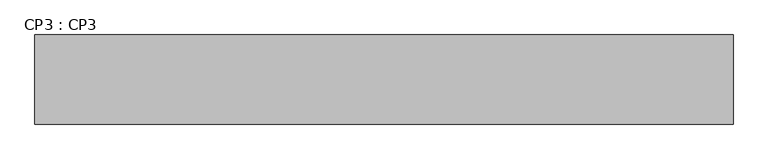
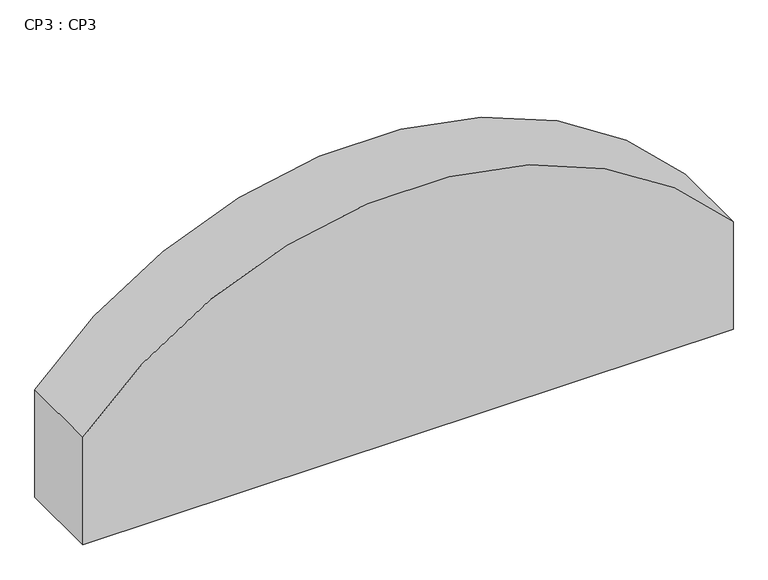
"""IFC4 building model written with IfcOpenShell, lengths in millimetres: beam geometry, CP3 : CP3."""

import ifcopenshell
import ifcopenshell.guid

model = None  # the IFC model being written
_history = None  # IfcOwnerHistory: only IFC2X3 demands one
_inside = {}  # id of a spatial element -> (the spatial element, [elements in it])
_under = {}  # id of a project, library or spatial element -> (it, [spatial elements below it])
_declared = {}  # id of a project -> (the project, [libraries it declares])
_typed = {}  # id of a type object -> (the type object, [elements of that type])
_made_of = {}  # id of a material, layer set ... -> (it, [elements and type objects made of it])


def new_model(schema):
    """Start an empty IFC model of exactly this schema.

    Asked for "IFC4X3", IfcOpenShell would pick the latest addendum, in which some entities
    have other attributes; the version numbers below select the first issue.
    IFC2X3 requires an IfcOwnerHistory on every rooted entity: one is made here for all.
    """
    global model, _history
    if schema == "IFC4X3":
        model = ifcopenshell.file(schema_version=(4, 3, 0, 0))
    else:
        model = ifcopenshell.file(schema=schema)
    _inside.clear()
    _under.clear()
    _declared.clear()
    _typed.clear()
    _made_of.clear()
    _history = None
    if model.schema == "IFC2X3":
        org = make("IfcOrganization", Name="unknown")
        user = make(
            "IfcPersonAndOrganization",
            ThePerson=make("IfcPerson", FamilyName="unknown"),
            TheOrganization=org,
        )
        app = make(
            "IfcApplication",
            ApplicationDeveloper=org,
            Version="unknown",
            ApplicationFullName="unknown",
            ApplicationIdentifier="unknown",
        )
        _history = make(
            "IfcOwnerHistory",
            OwningUser=user,
            OwningApplication=app,
            ChangeAction="ADDED",
            CreationDate=0,
        )
    return model


def make(cls, **values):
    """One entity of the class cls with the attributes given. An attribute that is None is left unset."""
    return model.create_entity(
        cls, **{name: value for name, value in values.items() if value is not None}
    )


def rooted(cls, **values):
    """An entity with a GlobalId (a new one), such as an element, a storey or a relation."""
    return make(cls, GlobalId=ifcopenshell.guid.new(), OwnerHistory=_history, **values)


def si_unit(unit_type, name, prefix=None):
    """IfcSIUnit, for example si_unit("LENGTHUNIT", "METRE", prefix="MILLI")."""
    return make("IfcSIUnit", UnitType=unit_type, Prefix=prefix, Name=name)


def assignment(units):
    """IfcUnitAssignment: the units of a project."""
    return None if units is None else make("IfcUnitAssignment", Units=units)


def point(xyz):
    """IfcCartesianPoint."""
    return None if xyz is None else make("IfcCartesianPoint", Coordinates=xyz)


def direction(xyz):
    """IfcDirection."""
    return None if xyz is None else make("IfcDirection", DirectionRatios=xyz)


def frame(location, z_axis=None, x_axis=None):
    """IfcAxis2Placement3D, a coordinate frame: its origin and axes. An axis left out is left unset."""
    return make(
        "IfcAxis2Placement3D",
        Location=point(location),
        Axis=direction(z_axis),
        RefDirection=direction(x_axis),
    )


def frame_2d(location, x_axis=None):
    """IfcAxis2Placement2D, a coordinate frame in the plane: its origin and x axis."""
    return make(
        "IfcAxis2Placement2D", Location=point(location), RefDirection=direction(x_axis)
    )


def origin():
    """The frame at (0, 0, 0) with its axes left unset."""
    return frame((0.0, 0.0, 0.0))


def place(relative_to, where):
    """IfcLocalPlacement: puts the frame where relative to a parent placement (None: the world)."""
    return make(
        "IfcLocalPlacement", PlacementRelTo=relative_to, RelativePlacement=where
    )


def context(
    kind, dimensions, precision=None, world=None, true_north=None, identifier=None
):
    """IfcGeometricRepresentationContext, for example the 3D "Model" context."""
    return make(
        "IfcGeometricRepresentationContext",
        ContextIdentifier=identifier,
        ContextType=kind,
        CoordinateSpaceDimension=dimensions,
        Precision=precision,
        WorldCoordinateSystem=world,
        TrueNorth=true_north,
    )


def project(units=None, contexts=None):
    """IfcProject with its units and contexts."""
    return rooted(
        "IfcProject",
        Name="project",
        RepresentationContexts=contexts,
        UnitsInContext=assignment(units),
    )


def spatial(cls, under=None, at=None, **own):
    """A site, building, storey or space (cls), placed at a placement, below another one or the project."""
    s = rooted(cls, ObjectPlacement=at, **own)
    if under is not None:
        _under.setdefault(under.id(), (under, []))[1].append(s)
    return s


def polyline(points):
    """IfcPolyline through the points."""
    return make("IfcPolyline", Points=[point(p) for p in points])


def circle_curve(where, radius):
    """IfcCircle in the frame where."""
    return make("IfcCircle", Position=where, Radius=radius)


def trimmed(basis, trim1, trim2, sense, master):
    """IfcTrimmedCurve: the piece of a basis curve between two trims."""
    return make(
        "IfcTrimmedCurve",
        BasisCurve=basis,
        Trim1=trim1,
        Trim2=trim2,
        SenseAgreement=sense,
        MasterRepresentation=master,
    )


def segment(curve, same_sense, transition):
    """IfcCompositeCurveSegment."""
    return make(
        "IfcCompositeCurveSegment",
        Transition=transition,
        SameSense=same_sense,
        ParentCurve=curve,
    )


def composite_curve(segments, self_intersect=None):
    """IfcCompositeCurve: segments joined end to end."""
    return make("IfcCompositeCurve", Segments=segments, SelfIntersect=self_intersect)


def outline(outer, holes=None, kind="AREA"):
    """IfcArbitraryClosedProfileDef: a profile drawn as a closed curve; with holes, ...WithVoids."""
    if holes is None:
        return make("IfcArbitraryClosedProfileDef", ProfileType=kind, OuterCurve=outer)
    return make(
        "IfcArbitraryProfileDefWithVoids",
        ProfileType=kind,
        OuterCurve=outer,
        InnerCurves=holes,
    )


def extrude(swept, where, along, depth):
    """IfcExtrudedAreaSolid: the profile swept, set in the frame where, extruded along a direction by depth."""
    return make(
        "IfcExtrudedAreaSolid",
        SweptArea=swept,
        Position=where,
        ExtrudedDirection=direction(along),
        Depth=depth,
    )


def shape(context_of_items, identifier, shape_type, items):
    """IfcShapeRepresentation: the items that make up one representation, for example the "Body"."""
    return make(
        "IfcShapeRepresentation",
        ContextOfItems=context_of_items,
        RepresentationIdentifier=identifier,
        RepresentationType=shape_type,
        Items=items,
    )


def source(mapping_origin, context_of_items, identifier, shape_type, items):
    """IfcRepresentationMap: a shape defined once, which mapped items show again and again."""
    return make(
        "IfcRepresentationMap",
        MappingOrigin=mapping_origin,
        MappedRepresentation=shape(context_of_items, identifier, shape_type, items),
    )


def transform(
    local_origin,
    x_axis=None,
    y_axis=None,
    z_axis=None,
    scale=None,
    scale2=None,
    scale3=None,
    uniform=True,
):
    """IfcCartesianTransformationOperator3D, or its non-uniform kind. x_axis, y_axis, z_axis: its Axis1, 2, 3."""
    if uniform:
        return make(
            "IfcCartesianTransformationOperator3D",
            Axis1=direction(x_axis),
            Axis2=direction(y_axis),
            LocalOrigin=point(local_origin),
            Scale=scale,
            Axis3=direction(z_axis),
        )
    return make(
        "IfcCartesianTransformationOperator3DnonUniform",
        Axis1=direction(x_axis),
        Axis2=direction(y_axis),
        LocalOrigin=point(local_origin),
        Scale=scale,
        Axis3=direction(z_axis),
        Scale2=scale2,
        Scale3=scale3,
    )


def mapped(mapping_source, mapping_target):
    """IfcMappedItem: shows the shape of a source again, moved by a transform."""
    return make(
        "IfcMappedItem", MappingSource=mapping_source, MappingTarget=mapping_target
    )


def made_of(thing, what):
    """Note that an element or type object is made of a material, layer set ...; save() writes the relation."""
    if what is not None:
        _made_of.setdefault(what.id(), (what, []))[1].append(thing)
    return thing


def element(
    cls,
    number,
    at=None,
    inside=None,
    cuts=None,
    type_object=None,
    material=None,
    context=None,
    identifier="Body",
    shape_type=None,
    held_by="IfcProductDefinitionShape",
    body=None,
    shapes=None,
    **own,
):
    """One element of the class cls, such as IfcWall. Its Tag is "e" and its number.

    at: its placement. inside: the storey or other place that contains it. cuts: it is an
    opening in that element (IfcRelVoidsElement). A single representation is given by context,
    identifier, shape_type and body (its items); several are given by shapes. held_by: the class
    of the entity that holds the representations. save() writes the other relations.
    """
    e = rooted(cls, Tag="e%d" % number, ObjectPlacement=at, **own)
    if body is not None:
        shapes = [shape(context, identifier, shape_type, body)]
    if shapes is not None:
        e.Representation = make(held_by, Representations=shapes)
    if inside is not None:
        _inside.setdefault(inside.id(), (inside, []))[1].append(e)
    if cuts is not None:
        rooted(
            "IfcRelVoidsElement", RelatingBuildingElement=cuts, RelatedOpeningElement=e
        )
    if type_object is not None:
        _typed.setdefault(type_object.id(), (type_object, []))[1].append(e)
    return made_of(e, material)


def aggregate(whole, parts):
    """IfcRelAggregates: a whole, such as a stair, and the parts it consists of."""
    return rooted("IfcRelAggregates", RelatingObject=whole, RelatedObjects=parts)


def save(model, path):
    """Write the relations noted so far, then the file.

    IfcRelAggregates (storeys below a building ...), IfcRelContainedInSpatialStructure (elements
    in a storey), IfcRelDefinesByType, IfcRelAssociatesMaterial and IfcRelDeclares: one each for
    every whole, place, type object, material and project.
    """
    for whole, parts in _under.values():
        aggregate(whole, parts)
    for where, things in _inside.values():
        rooted(
            "IfcRelContainedInSpatialStructure",
            RelatedElements=things,
            RelatingStructure=where,
        )
    for kind, things in _typed.values():
        rooted("IfcRelDefinesByType", RelatedObjects=things, RelatingType=kind)
    for what, things in _made_of.values():
        rooted("IfcRelAssociatesMaterial", RelatedObjects=things, RelatingMaterial=what)
    for by, libraries in _declared.values():
        rooted("IfcRelDeclares", RelatingContext=by, RelatedDefinitions=libraries)
    model.write(path)


def cp3_cp3_3d258a3e(model_context):
    return source(origin(), model_context, "Body", "SweptSolid", [
        extrude(outline(composite_curve([segment(trimmed(circle_curve(frame_2d((12603.2870371, 37833.2245514)), 3096.7129629), [point((14620.0, 40183.2245513))], [point((14620.0, 35483.2245514))], False, "CARTESIAN"), True, "CONTINUOUS"), segment(polyline([(14620.0, 35483.2245514), (13800.0, 35483.2245514), (13800.0, 40183.2245513), (14620.0, 40183.2245513)]), True, "CONTINUOUS")], self_intersect=False)), frame((0.0, -100.2551788, 0.0), z_axis=(0.0, 1.0, 0.0), x_axis=(0.0, 0.0, 1.0)), (0.0, 0.0, 1.0), 599.9551778),
    ])


if __name__ == "__main__":
    model = new_model("IFC4")
    model_context = context("Model", 3, world=origin())
    ifc_project = project(units=[si_unit("LENGTHUNIT", "METRE", prefix="MILLI")], contexts=[model_context])
    site = spatial("IfcSite", under=ifc_project)
    building = spatial("IfcBuilding", under=site)
    placement = place(None, origin())
    cp3_cp3_shape = cp3_cp3_3d258a3e(model_context)
    element("IfcBeam", 1, ObjectType="CP3 : CP3", at=placement, inside=building, context=model_context, shape_type="MappedRepresentation", body=[
        mapped(cp3_cp3_shape, transform((0.0, 0.0, 0.0), x_axis=(1.0, 0.0, 0.0), y_axis=(0.0, 1.0, 0.0), z_axis=(0.0, 0.0, 1.0))),
    ])
    save(model, "model.ifc")
